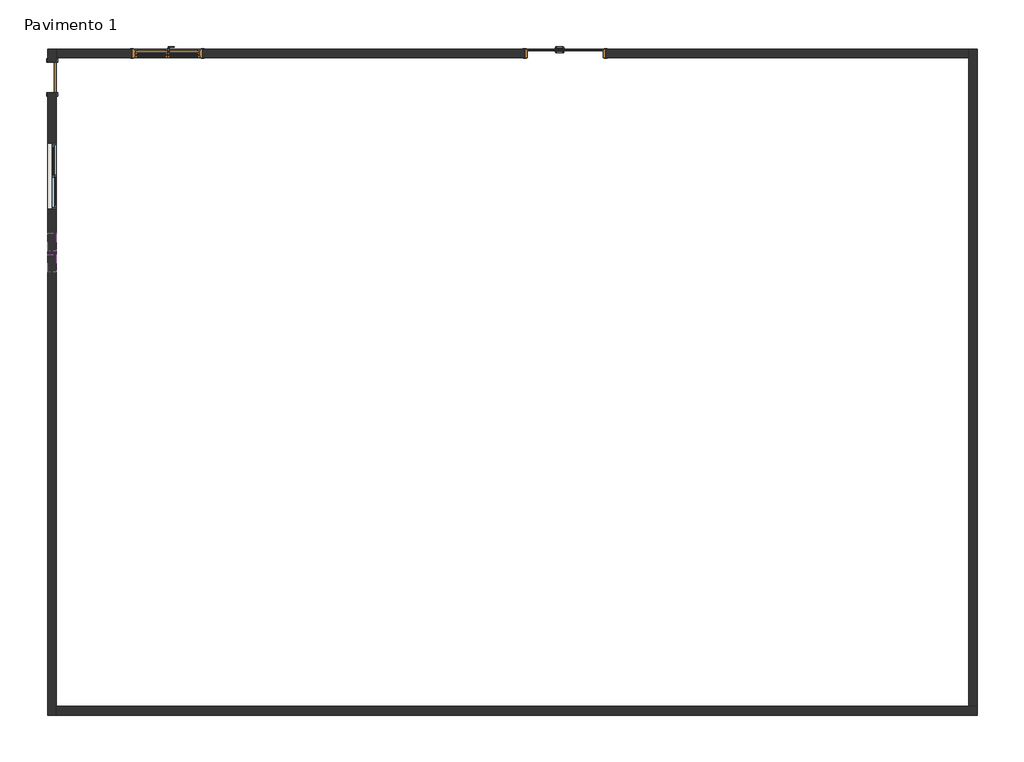
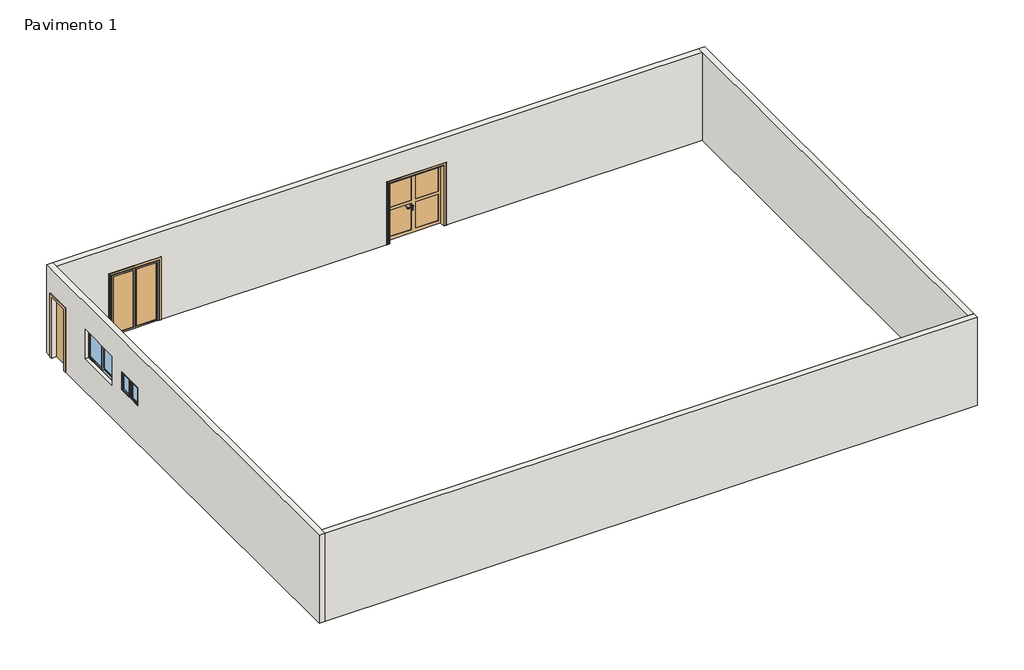
# One storey: 4 walls, 3 doors, 3 windows.
"""IFC4 building model written with IfcOpenShell, lengths in millimetres."""

import ifcopenshell
import ifcopenshell.guid

model = None  # the IFC model being written
_history = None  # IfcOwnerHistory: only IFC2X3 demands one
_inside = {}  # id of a spatial element -> (the spatial element, [elements in it])
_under = {}  # id of a project, library or spatial element -> (it, [spatial elements below it])
_declared = {}  # id of a project -> (the project, [libraries it declares])
_typed = {}  # id of a type object -> (the type object, [elements of that type])
_made_of = {}  # id of a material, layer set ... -> (it, [elements and type objects made of it])


def new_model(schema):
    """Start an empty IFC model of exactly this schema.

    Asked for "IFC4X3", IfcOpenShell would pick the latest addendum, in which some entities
    have other attributes; the version numbers below select the first issue.
    IFC2X3 requires an IfcOwnerHistory on every rooted entity: one is made here for all.
    """
    global model, _history
    if schema == "IFC4X3":
        model = ifcopenshell.file(schema_version=(4, 3, 0, 0))
    else:
        model = ifcopenshell.file(schema=schema)
    _inside.clear()
    _under.clear()
    _declared.clear()
    _typed.clear()
    _made_of.clear()
    _history = None
    if model.schema == "IFC2X3":
        org = make("IfcOrganization", Name="unknown")
        user = make(
            "IfcPersonAndOrganization",
            ThePerson=make("IfcPerson", FamilyName="unknown"),
            TheOrganization=org,
        )
        app = make(
            "IfcApplication",
            ApplicationDeveloper=org,
            Version="unknown",
            ApplicationFullName="unknown",
            ApplicationIdentifier="unknown",
        )
        _history = make(
            "IfcOwnerHistory",
            OwningUser=user,
            OwningApplication=app,
            ChangeAction="ADDED",
            CreationDate=0,
        )
    return model


def make(cls, **values):
    """One entity of the class cls with the attributes given. An attribute that is None is left unset."""
    return model.create_entity(
        cls, **{name: value for name, value in values.items() if value is not None}
    )


def rooted(cls, **values):
    """An entity with a GlobalId (a new one), such as an element, a storey or a relation."""
    return make(cls, GlobalId=ifcopenshell.guid.new(), OwnerHistory=_history, **values)


def si_unit(unit_type, name, prefix=None):
    """IfcSIUnit, for example si_unit("LENGTHUNIT", "METRE", prefix="MILLI")."""
    return make("IfcSIUnit", UnitType=unit_type, Prefix=prefix, Name=name)


def assignment(units):
    """IfcUnitAssignment: the units of a project."""
    return None if units is None else make("IfcUnitAssignment", Units=units)


def point(xyz):
    """IfcCartesianPoint."""
    return None if xyz is None else make("IfcCartesianPoint", Coordinates=xyz)


def direction(xyz):
    """IfcDirection."""
    return None if xyz is None else make("IfcDirection", DirectionRatios=xyz)


def frame(location, z_axis=None, x_axis=None):
    """IfcAxis2Placement3D, a coordinate frame: its origin and axes. An axis left out is left unset."""
    return make(
        "IfcAxis2Placement3D",
        Location=point(location),
        Axis=direction(z_axis),
        RefDirection=direction(x_axis),
    )


def frame_2d(location, x_axis=None):
    """IfcAxis2Placement2D, a coordinate frame in the plane: its origin and x axis."""
    return make(
        "IfcAxis2Placement2D", Location=point(location), RefDirection=direction(x_axis)
    )


def origin():
    """The frame at (0, 0, 0) with its axes left unset."""
    return frame((0.0, 0.0, 0.0))


def origin_with_axes():
    """The frame at (0, 0, 0) with the z axis (0, 0, 1) and the x axis (1, 0, 0) written out."""
    return frame((0.0, 0.0, 0.0), z_axis=(0.0, 0.0, 1.0), x_axis=(1.0, 0.0, 0.0))


def place(relative_to, where):
    """IfcLocalPlacement: puts the frame where relative to a parent placement (None: the world)."""
    return make(
        "IfcLocalPlacement", PlacementRelTo=relative_to, RelativePlacement=where
    )


def context(
    kind, dimensions, precision=None, world=None, true_north=None, identifier=None
):
    """IfcGeometricRepresentationContext, for example the 3D "Model" context."""
    return make(
        "IfcGeometricRepresentationContext",
        ContextIdentifier=identifier,
        ContextType=kind,
        CoordinateSpaceDimension=dimensions,
        Precision=precision,
        WorldCoordinateSystem=world,
        TrueNorth=true_north,
    )


def project(units=None, contexts=None):
    """IfcProject with its units and contexts."""
    return rooted(
        "IfcProject",
        Name="project",
        RepresentationContexts=contexts,
        UnitsInContext=assignment(units),
    )


def spatial(cls, under=None, at=None, **own):
    """A site, building, storey or space (cls), placed at a placement, below another one or the project."""
    s = rooted(cls, ObjectPlacement=at, **own)
    if under is not None:
        _under.setdefault(under.id(), (under, []))[1].append(s)
    return s


def polyline(points):
    """IfcPolyline through the points."""
    return make("IfcPolyline", Points=[point(p) for p in points])


def circle_curve(where, radius):
    """IfcCircle in the frame where."""
    return make("IfcCircle", Position=where, Radius=radius)


def ellipse_curve(where, semi_axis1, semi_axis2):
    """IfcEllipse in the frame where."""
    return make(
        "IfcEllipse", Position=where, SemiAxis1=semi_axis1, SemiAxis2=semi_axis2
    )


def trimmed(basis, trim1, trim2, sense, master):
    """IfcTrimmedCurve: the piece of a basis curve between two trims."""
    return make(
        "IfcTrimmedCurve",
        BasisCurve=basis,
        Trim1=trim1,
        Trim2=trim2,
        SenseAgreement=sense,
        MasterRepresentation=master,
    )


def segment(curve, same_sense, transition):
    """IfcCompositeCurveSegment."""
    return make(
        "IfcCompositeCurveSegment",
        Transition=transition,
        SameSense=same_sense,
        ParentCurve=curve,
    )


def composite_curve(segments, self_intersect=None):
    """IfcCompositeCurve: segments joined end to end."""
    return make("IfcCompositeCurve", Segments=segments, SelfIntersect=self_intersect)


def outline(outer, holes=None, kind="AREA"):
    """IfcArbitraryClosedProfileDef: a profile drawn as a closed curve; with holes, ...WithVoids."""
    if holes is None:
        return make("IfcArbitraryClosedProfileDef", ProfileType=kind, OuterCurve=outer)
    return make(
        "IfcArbitraryProfileDefWithVoids",
        ProfileType=kind,
        OuterCurve=outer,
        InnerCurves=holes,
    )


def extrude(swept, where, along, depth):
    """IfcExtrudedAreaSolid: the profile swept, set in the frame where, extruded along a direction by depth."""
    return make(
        "IfcExtrudedAreaSolid",
        SweptArea=swept,
        Position=where,
        ExtrudedDirection=direction(along),
        Depth=depth,
    )


def faces_of(points, faces, orient=None, outer=None):
    """IfcFace entities. A face is a list of loops; a loop is a list of indices into points, from 0.

    orient and outer hold one flag for each loop. By default every Orientation is true, the
    first loop of a face is its IfcFaceOuterBound and the others are IfcFaceBound.
    """
    made = []
    for i, loops in enumerate(faces):
        bounds = []
        for j, loop in enumerate(loops):
            is_outer = j == 0 if outer is None else outer[i][j]
            bounds.append(
                make(
                    "IfcFaceOuterBound" if is_outer else "IfcFaceBound",
                    Bound=make("IfcPolyLoop", Polygon=[points[k] for k in loop]),
                    Orientation=True if orient is None else orient[i][j],
                )
            )
        made.append(make("IfcFace", Bounds=bounds))
    return made


def faceted_brep(points, faces, orient=None, outer=None, voids=None):
    """IfcFacetedBrep: a solid bounded by flat faces; with voids (closed shells), ...WithVoids."""
    shared = [point(p) for p in points]
    hull = make("IfcClosedShell", CfsFaces=faces_of(shared, faces, orient, outer))
    if voids is None:
        return make("IfcFacetedBrep", Outer=hull)
    return make(
        "IfcFacetedBrepWithVoids",
        Outer=hull,
        Voids=[
            make(cls, CfsFaces=faces_of(shared, fs, o, b)) for cls, fs, o, b in voids
        ],
    )


def shape(context_of_items, identifier, shape_type, items):
    """IfcShapeRepresentation: the items that make up one representation, for example the "Body"."""
    return make(
        "IfcShapeRepresentation",
        ContextOfItems=context_of_items,
        RepresentationIdentifier=identifier,
        RepresentationType=shape_type,
        Items=items,
    )


def source(mapping_origin, context_of_items, identifier, shape_type, items):
    """IfcRepresentationMap: a shape defined once, which mapped items show again and again."""
    return make(
        "IfcRepresentationMap",
        MappingOrigin=mapping_origin,
        MappedRepresentation=shape(context_of_items, identifier, shape_type, items),
    )


def transform(
    local_origin,
    x_axis=None,
    y_axis=None,
    z_axis=None,
    scale=None,
    scale2=None,
    scale3=None,
    uniform=True,
):
    """IfcCartesianTransformationOperator3D, or its non-uniform kind. x_axis, y_axis, z_axis: its Axis1, 2, 3."""
    if uniform:
        return make(
            "IfcCartesianTransformationOperator3D",
            Axis1=direction(x_axis),
            Axis2=direction(y_axis),
            LocalOrigin=point(local_origin),
            Scale=scale,
            Axis3=direction(z_axis),
        )
    return make(
        "IfcCartesianTransformationOperator3DnonUniform",
        Axis1=direction(x_axis),
        Axis2=direction(y_axis),
        LocalOrigin=point(local_origin),
        Scale=scale,
        Axis3=direction(z_axis),
        Scale2=scale2,
        Scale3=scale3,
    )


def mapped(mapping_source, mapping_target):
    """IfcMappedItem: shows the shape of a source again, moved by a transform."""
    return make(
        "IfcMappedItem", MappingSource=mapping_source, MappingTarget=mapping_target
    )


def made_of(thing, what):
    """Note that an element or type object is made of a material, layer set ...; save() writes the relation."""
    if what is not None:
        _made_of.setdefault(what.id(), (what, []))[1].append(thing)
    return thing


def element(
    cls,
    number,
    at=None,
    inside=None,
    cuts=None,
    type_object=None,
    material=None,
    context=None,
    identifier="Body",
    shape_type=None,
    held_by="IfcProductDefinitionShape",
    body=None,
    shapes=None,
    **own,
):
    """One element of the class cls, such as IfcWall. Its Tag is "e" and its number.

    at: its placement. inside: the storey or other place that contains it. cuts: it is an
    opening in that element (IfcRelVoidsElement). A single representation is given by context,
    identifier, shape_type and body (its items); several are given by shapes. held_by: the class
    of the entity that holds the representations. save() writes the other relations.
    """
    e = rooted(cls, Tag="e%d" % number, ObjectPlacement=at, **own)
    if body is not None:
        shapes = [shape(context, identifier, shape_type, body)]
    if shapes is not None:
        e.Representation = make(held_by, Representations=shapes)
    if inside is not None:
        _inside.setdefault(inside.id(), (inside, []))[1].append(e)
    if cuts is not None:
        rooted(
            "IfcRelVoidsElement", RelatingBuildingElement=cuts, RelatedOpeningElement=e
        )
    if type_object is not None:
        _typed.setdefault(type_object.id(), (type_object, []))[1].append(e)
    return made_of(e, material)


def aggregate(whole, parts):
    """IfcRelAggregates: a whole, such as a stair, and the parts it consists of."""
    return rooted("IfcRelAggregates", RelatingObject=whole, RelatedObjects=parts)


def save(model, path):
    """Write the relations noted so far, then the file.

    IfcRelAggregates (storeys below a building ...), IfcRelContainedInSpatialStructure (elements
    in a storey), IfcRelDefinesByType, IfcRelAssociatesMaterial and IfcRelDeclares: one each for
    every whole, place, type object, material and project.
    """
    for whole, parts in _under.values():
        aggregate(whole, parts)
    for where, things in _inside.values():
        rooted(
            "IfcRelContainedInSpatialStructure",
            RelatedElements=things,
            RelatingStructure=where,
        )
    for kind, things in _typed.values():
        rooted("IfcRelDefinesByType", RelatedObjects=things, RelatingType=kind)
    for what, things in _made_of.values():
        rooted("IfcRelAssociatesMaterial", RelatedObjects=things, RelatingMaterial=what)
    for by, libraries in _declared.values():
        rooted("IfcRelDeclares", RelatingContext=by, RelatedDefinitions=libraries)
    model.write(path)


def plane_surface(at):
    """IfcPlane: the flat surface through the origin of the frame at, square to its z axis."""
    return make("IfcPlane", Position=at)


def cylinder_surface(at, radius):
    """IfcCylindricalSurface: all points at the distance radius from the z axis of the frame at."""
    return make("IfcCylindricalSurface", Position=at, Radius=radius)


def revolved_surface(curve, axis_point, axis_direction):
    """IfcSurfaceOfRevolution: the curve turned about the line through axis_point along axis_direction."""
    return make(
        "IfcSurfaceOfRevolution",
        SweptCurve=make("IfcArbitraryOpenProfileDef", ProfileType="CURVE", Curve=curve),
        AxisPosition=make("IfcAxis1Placement", Location=point(axis_point), Axis=direction(axis_direction)),
    )


def advanced_brep(points, edges, surfaces, faces):
    """IfcAdvancedBrep: a solid bounded by faces that lie on surfaces and meet in shared edges.

    An edge is (start, end): straight between two places in points (the first is 0);
    or (start, end, curve); or (start, end, curve, False) where it runs against its curve.
    A face is (place in surfaces, loops), or (place, loops, False) where it looks against
    its surface's normal. A loop lists edges by number (the first is 1), with a minus sign
    where the edge is run from its end to its start. The first loop is the outer one.
    """
    corners = [point(p) for p in points]
    vertices = [make("IfcVertexPoint", VertexGeometry=c) for c in corners]
    made = []
    for start, end, *more in edges:
        made.append(
            make(
                "IfcEdgeCurve",
                EdgeStart=vertices[start],
                EdgeEnd=vertices[end],
                EdgeGeometry=more[0] if more else make("IfcPolyline", Points=[corners[start], corners[end]]),
                SameSense=more[1] if len(more) > 1 else True,
            )
        )
    hull = []
    for where, loops, *sense in faces:
        bounds = []
        for j, loop in enumerate(loops):
            ring = [make("IfcOrientedEdge", EdgeElement=made[abs(k) - 1], Orientation=k > 0) for k in loop]
            bounds.append(
                make(
                    "IfcFaceOuterBound" if j == 0 else "IfcFaceBound",
                    Bound=make("IfcEdgeLoop", EdgeList=ring),
                    Orientation=True,
                )
            )
        hull.append(make("IfcAdvancedFace", Bounds=bounds, FaceSurface=surfaces[where], SameSense=sense[0] if sense else True))
    return make("IfcAdvancedBrep", Outer=make("IfcClosedShell", CfsFaces=hull))


def porta_210x070_b827da78(model_context):
    return source(origin(), model_context, "Body", "SweptSolid", [
        extrude(outline(polyline([(2176.0, -426.0), (0.0, -426.0), (0.0, -350.0), (2100.0, -350.0), (2100.0, 350.0), (0.0, 350.0), (0.0, 426.0), (2176.0, 426.0), (2176.0, -426.0)])), frame((0.0, -125.0, 0.0), z_axis=(0.0, 1.0, 0.0), x_axis=(0.0, 0.0, 1.0)), (0.0, 0.0, 1.0), 25.0),
        extrude(outline(polyline([(2176.0, 426.0), (2176.0, -426.0), (0.0, -426.0), (0.0, -350.0), (2100.0, -350.0), (2100.0, 350.0), (0.0, 350.0), (0.0, 426.0), (2176.0, 426.0)])), frame((0.0, 100.0, 0.0), z_axis=(0.0, 1.0, 0.0), x_axis=(0.0, 0.0, 1.0)), (0.0, 0.0, 1.0), 25.0),
        extrude(outline(polyline([(350.0, -49.0), (350.0, -100.0), (-350.0, -100.0), (-350.0, -49.0), (350.0, -49.0)])), origin_with_axes(), (0.0, 0.0, 1.0), 2100.0),
    ])


def porta_160x210_6cb1d5fe(model_context):
    return source(origin(), model_context, "Body", "SolidModel", [
        extrude(outline(polyline([(-680.0, -7.0), (-680.0, 7.0), (-50.0, 7.0), (-50.0, -7.0), (-680.0, -7.0)])), frame((0.0, 0.0, 50.0), z_axis=(0.0, 0.0, 1.0), x_axis=(1.0, 0.0, 0.0)), (0.0, 0.0, 1.0), 1930.0),
        extrude(outline(polyline([(2030.0, -730.0), (0.0, -730.0), (0.0, 0.0), (2030.0, 0.0), (2030.0, -730.0)]), holes=[polyline([(50.0, -680.0), (1980.0, -680.0), (1980.0, -50.0), (50.0, -50.0), (50.0, -680.0)])]), frame((0.0, -20.0, 0.0), z_axis=(0.0, 1.0, 0.0), x_axis=(0.0, 0.0, 1.0)), (0.0, 0.0, 1.0), 40.0),
        extrude(outline(polyline([(680.0, -7.0), (50.0, -7.0), (50.0, 7.0), (680.0, 7.0), (680.0, -7.0)])), frame((0.0, 0.0, 50.0), z_axis=(0.0, 0.0, 1.0), x_axis=(1.0, 0.0, 0.0)), (0.0, 0.0, 1.0), 1930.0),
        extrude(outline(polyline([(2030.0, 730.0), (2030.0, 0.0), (0.0, 0.0), (0.0, 730.0), (2030.0, 730.0)]), holes=[polyline([(50.0, 680.0), (50.0, 50.0), (1980.0, 50.0), (1980.0, 680.0), (50.0, 680.0)])]), frame((0.0, -20.0, 0.0), z_axis=(0.0, 1.0, 0.0), x_axis=(0.0, 0.0, 1.0)), (0.0, 0.0, 1.0), 40.0),
        extrude(outline(polyline([(-50.0, 89.0), (-50.0, 65.0), (-687.0, 65.0), (-687.0, 89.0), (-50.0, 89.0)])), frame((0.0, 0.0, 53.0), z_axis=(0.0, 0.0, 1.0), x_axis=(1.0, 0.0, 0.0)), (0.0, 0.0, 1.0), 1934.0),
        extrude(outline(polyline([(2037.0, -737.0), (3.0, -737.0), (3.0, 0.0), (2037.0, 0.0), (2037.0, -737.0)]), holes=[polyline([(53.0, -687.0), (1987.0, -687.0), (1987.0, -50.0), (53.0, -50.0), (53.0, -687.0)])]), frame((0.0, 57.0, 0.0), z_axis=(0.0, 1.0, 0.0), x_axis=(0.0, 0.0, 1.0)), (0.0, 0.0, 1.0), 40.0),
        extrude(outline(composite_curve([segment(trimmed(circle_curve(frame_2d((840.0, 25.0)), 15.0), [point((840.0, 40.0))], [point((840.0, 10.0))], False, "CARTESIAN"), True, "CONTINUOUS"), segment(trimmed(circle_curve(frame_2d((840.0, 25.0)), 15.0), [point((840.0, 10.0))], [point((840.0, 40.0))], False, "CARTESIAN"), True, "CONTINUOUS")], self_intersect=False)), frame((0.0, 107.0, 0.0), z_axis=(0.0, 1.0, 0.0), x_axis=(0.0, 0.0, 1.0)), (0.0, 0.0, 1.0), 10.0),
        extrude(outline(composite_curve([segment(trimmed(circle_curve(frame_2d((840.0, 25.0)), 15.0), [point((840.0, 40.0))], [point((840.0, 10.0))], False, "CARTESIAN"), True, "CONTINUOUS"), segment(trimmed(circle_curve(frame_2d((840.0, 25.0)), 15.0), [point((840.0, 10.0))], [point((840.0, 40.0))], False, "CARTESIAN"), True, "CONTINUOUS")], self_intersect=False)), frame((0.0, 37.0, 0.0), z_axis=(0.0, 1.0, 0.0), x_axis=(0.0, 0.0, 1.0)), (0.0, 0.0, 1.0), 10.0),
        extrude(outline(composite_curve([segment(trimmed(circle_curve(frame_2d((900.0, 25.0)), 8.0), [point((904.6523287, 18.4918637))], [point((900.0, 33.0))], False, "CARTESIAN"), True, "CONTINUOUS"), segment(trimmed(circle_curve(frame_2d((894.8738613, 50.3861901)), 18.1261387), [point((900.0, 33.0))], [point((913.0, 50.3861901))], True, "CARTESIAN"), True, "CONTINUOUS"), segment(polyline([(913.0, 50.3861901), (913.0, 126.6435909)]), True, "CONTINUOUS"), segment(trimmed(circle_curve(frame_2d((972.2709207, 123.0603388)), 59.3791355), [point((913.0, 126.6435909))], [point((922.2135558, 155.0))], False, "CARTESIAN"), True, "CONTINUOUS"), segment(polyline([(922.2135558, 155.0), (925.0, 155.0)]), True, "CONTINUOUS"), segment(trimmed(circle_curve(frame_2d((1003.2850638, 126.5772091)), 83.2850902), [point((925.0, 155.0))], [point((920.0, 126.6435909))], True, "CARTESIAN"), True, "CONTINUOUS"), segment(polyline([(920.0, 126.6435909), (920.0, 50.3674333)]), True, "CONTINUOUS"), segment(trimmed(circle_curve(frame_2d((882.7555521, 48.6675129)), 37.2832219), [point((920.0, 50.3674333))], [point((904.6523287, 18.4918637))], False, "CARTESIAN"), True, "CONTINUOUS")], self_intersect=False)), frame((0.0, 137.0, 0.0), z_axis=(0.0, 1.0, 0.0), x_axis=(0.0, 0.0, 1.0)), (0.0, 0.0, 1.0), 20.0),
        extrude(outline(composite_curve([segment(trimmed(circle_curve(frame_2d((894.8738682, 50.3861878)), 18.1261318), [point((899.9999903, 33.0))], [point((913.0, 50.3861878))], True, "CARTESIAN"), True, "CONTINUOUS"), segment(polyline([(913.0, 50.3861878), (913.0, 126.6435909)]), True, "CONTINUOUS"), segment(trimmed(circle_curve(frame_2d((972.2709207, 123.0603388)), 59.3791355), [point((913.0, 126.6435909))], [point((922.2135558, 155.0))], False, "CARTESIAN"), True, "CONTINUOUS"), segment(polyline([(922.2135558, 155.0), (925.0, 155.0)]), True, "CONTINUOUS"), segment(trimmed(circle_curve(frame_2d((1003.2850638, 126.5772091)), 83.2850902), [point((925.0, 155.0))], [point((920.0, 126.6435909))], True, "CARTESIAN"), True, "CONTINUOUS"), segment(polyline([(920.0, 126.6435909), (920.0, 50.3674333)]), True, "CONTINUOUS"), segment(trimmed(circle_curve(frame_2d((882.7555521, 48.6675129)), 37.2832219), [point((920.0, 50.3674333))], [point((904.6523287, 18.4918637))], False, "CARTESIAN"), True, "CONTINUOUS"), segment(trimmed(circle_curve(frame_2d((900.0, 25.0)), 8.0), [point((904.6523287, 18.4918637))], [point((899.9999903, 33.0))], False, "CARTESIAN"), True, "CONTINUOUS")], self_intersect=False)), frame((0.0, -3.0, 0.0), z_axis=(0.0, 1.0, 0.0), x_axis=(0.0, 0.0, 1.0)), (0.0, 0.0, 1.0), 20.0),
        extrude(outline(composite_curve([segment(trimmed(circle_curve(frame_2d((900.0, 25.0)), 8.0), [point((900.0, 33.0))], [point((900.0, 17.0))], False, "CARTESIAN"), True, "CONTINUOUS"), segment(trimmed(circle_curve(frame_2d((900.0, 25.0)), 8.0), [point((900.0, 17.0))], [point((900.0, 33.0))], False, "CARTESIAN"), True, "CONTINUOUS")], self_intersect=False)), frame((0.0, 107.0, 0.0), z_axis=(0.0, 1.0, 0.0), x_axis=(0.0, 0.0, 1.0)), (0.0, 0.0, 1.0), 30.0),
        extrude(outline(composite_curve([segment(trimmed(circle_curve(frame_2d((900.0, 25.0)), 8.0), [point((900.0, 33.0))], [point((900.0, 17.0))], False, "CARTESIAN"), True, "CONTINUOUS"), segment(trimmed(circle_curve(frame_2d((900.0, 25.0)), 8.0), [point((900.0, 17.0))], [point((900.0, 33.0))], False, "CARTESIAN"), True, "CONTINUOUS")], self_intersect=False)), frame((0.0, 17.0, 0.0), z_axis=(0.0, 1.0, 0.0), x_axis=(0.0, 0.0, 1.0)), (0.0, 0.0, 1.0), 30.0),
        extrude(outline(composite_curve([segment(trimmed(circle_curve(frame_2d((830.0, 25.0)), 25.0), [point((830.0, 0.0))], [point((830.0, 50.0))], False, "CARTESIAN"), True, "CONTINUOUS"), segment(polyline([(830.0, 50.0), (900.0, 50.0)]), True, "CONTINUOUS"), segment(trimmed(circle_curve(frame_2d((900.0, 25.0)), 25.0), [point((900.0, 50.0))], [point((900.0, 0.0))], False, "CARTESIAN"), True, "CONTINUOUS"), segment(polyline([(900.0, 0.0), (830.0, 0.0)]), True, "CONTINUOUS")], self_intersect=False)), frame((0.0, 97.0, 0.0), z_axis=(0.0, 1.0, 0.0), x_axis=(0.0, 0.0, 1.0)), (0.0, 0.0, 1.0), 10.0),
        extrude(outline(composite_curve([segment(trimmed(circle_curve(frame_2d((830.0, 25.0)), 25.0), [point((830.0, 0.0))], [point((830.0, 50.0))], False, "CARTESIAN"), True, "CONTINUOUS"), segment(polyline([(830.0, 50.0), (900.0, 50.0)]), True, "CONTINUOUS"), segment(trimmed(circle_curve(frame_2d((900.0, 25.0)), 25.0), [point((900.0, 50.0))], [point((900.0, 0.0))], False, "CARTESIAN"), True, "CONTINUOUS"), segment(polyline([(900.0, 0.0), (830.0, 0.0)]), True, "CONTINUOUS")], self_intersect=False)), frame((0.0, 47.0, 0.0), z_axis=(0.0, 1.0, 0.0), x_axis=(0.0, 0.0, 1.0)), (0.0, 0.0, 1.0), 10.0),
        extrude(outline(polyline([(50.0, 89.0), (687.0, 89.0), (687.0, 65.0), (50.0, 65.0), (50.0, 89.0)])), frame((0.0, 0.0, 53.0), z_axis=(0.0, 0.0, 1.0), x_axis=(1.0, 0.0, 0.0)), (0.0, 0.0, 1.0), 1934.0),
        extrude(outline(polyline([(2037.0, 737.0), (2037.0, 0.0), (3.0, 0.0), (3.0, 737.0), (2037.0, 737.0)]), holes=[polyline([(53.0, 687.0), (53.0, 50.0), (1987.0, 50.0), (1987.0, 687.0), (53.0, 687.0)])]), frame((0.0, 57.0, 0.0), z_axis=(0.0, 1.0, 0.0), x_axis=(0.0, 0.0, 1.0)), (0.0, 0.0, 1.0), 40.0),
        extrude(outline(polyline([(-50.0, -84.0), (-687.0, -84.0), (-687.0, -70.0), (-50.0, -70.0), (-50.0, -84.0)])), frame((0.0, 0.0, 53.0), z_axis=(0.0, 0.0, 1.0), x_axis=(1.0, 0.0, 0.0)), (0.0, 0.0, 1.0), 1934.0),
        extrude(outline(polyline([(3.0, -737.0), (3.0, 0.0), (2037.0, 0.0), (2037.0, -737.0), (3.0, -737.0)]), holes=[polyline([(1987.0, -687.0), (1987.0, -50.0), (53.0, -50.0), (53.0, -687.0), (1987.0, -687.0)])]), frame((0.0, -97.0, 0.0), z_axis=(0.0, 1.0, 0.0), x_axis=(0.0, 0.0, 1.0)), (0.0, 0.0, 1.0), 40.0),
        extrude(outline(polyline([(50.0, -84.0), (50.0, -70.0), (687.0, -70.0), (687.0, -84.0), (50.0, -84.0)])), frame((0.0, 0.0, 53.0), z_axis=(0.0, 0.0, 1.0), x_axis=(1.0, 0.0, 0.0)), (0.0, 0.0, 1.0), 1934.0),
        extrude(outline(polyline([(3.0, 737.0), (2037.0, 737.0), (2037.0, 0.0), (3.0, 0.0), (3.0, 737.0)]), holes=[polyline([(1987.0, 687.0), (53.0, 687.0), (53.0, 50.0), (1987.0, 50.0), (1987.0, 687.0)])]), frame((0.0, -97.0, 0.0), z_axis=(0.0, 1.0, 0.0), x_axis=(0.0, 0.0, 1.0)), (0.0, 0.0, 1.0), 40.0),
        faceted_brep([(-740.0, -100.0, 0.0), (-800.0, -100.0, 0.0), (-800.0, 100.0, 0.0), (-740.0, 100.0, 0.0), (-740.0, 54.0, 0.0), (-730.0, 54.0, 0.0), (-730.0, -54.0, 0.0), (-740.0, -54.0, 0.0), (-740.0, -100.0, 2040.0), (740.0, -100.0, 2040.0), (740.0, -100.0, 0.0), (800.0, -100.0, 0.0), (800.0, -100.0, 2100.0), (-800.0, -100.0, 2100.0), (-800.0, 100.0, 2100.0), (800.0, 100.0, 2100.0), (800.0, 100.0, 0.0), (740.0, 100.0, 0.0), (740.0, 100.0, 2040.0), (-740.0, 100.0, 2040.0), (-740.0, 54.0, 2040.0), (740.0, 54.0, 2040.0), (740.0, 54.0, 0.0), (730.0, 54.0, 0.0), (730.0, 54.0, 2030.0), (-730.0, 54.0, 2030.0), (-730.0, -54.0, 2030.0), (730.0, -54.0, 2030.0), (730.0, -54.0, 0.0), (740.0, -54.0, 0.0), (740.0, -54.0, 2040.0), (-740.0, -54.0, 2040.0)], [[[0, 1, 2, 3, 4, 5, 6, 7]], [[1, 0, 8, 9, 10, 11, 12, 13]], [[2, 1, 13, 14]], [[3, 2, 14, 15, 16, 17, 18, 19]], [[4, 3, 19, 20]], [[5, 4, 20, 21, 22, 23, 24, 25]], [[6, 5, 25, 26]], [[7, 6, 26, 27, 28, 29, 30, 31]], [[0, 7, 31, 8]], [[10, 29, 28, 23, 22, 17, 16, 11]], [[9, 30, 29, 10]], [[27, 24, 23, 28]], [[21, 18, 17, 22]], [[15, 12, 11, 16]], [[14, 13, 12, 15]], [[20, 19, 18, 21]], [[26, 25, 24, 27]], [[8, 31, 30, 9]]]),
        faceted_brep([(843.0, -104.0, 0.0), (837.0, -110.0, 0.0), (773.0, -110.0, 0.0), (773.0, -100.0, 0.0), (843.0, -100.0, 0.0), (843.0, -104.0, 2143.0), (837.0, -110.0, 2137.0), (-837.0, -110.0, 2137.0), (-837.0, -110.0, 0.0), (-773.0, -110.0, 0.0), (-773.0, -110.0, 2073.0), (773.0, -110.0, 2073.0), (773.0, -100.0, 2073.0), (-773.0, -100.0, 2073.0), (-773.0, -100.0, 0.0), (-843.0, -100.0, 0.0), (-843.0, -100.0, 2143.0), (843.0, -100.0, 2143.0), (-843.0, -104.0, 0.0), (-843.0, -104.0, 2143.0)], [[[0, 1, 2, 3, 4]], [[1, 0, 5, 6]], [[2, 1, 6, 7, 8, 9, 10, 11]], [[3, 2, 11, 12]], [[4, 3, 12, 13, 14, 15, 16, 17]], [[0, 4, 17, 5]], [[18, 15, 14, 9, 8]], [[19, 16, 15, 18]], [[13, 10, 9, 14]], [[7, 19, 18, 8]], [[6, 5, 19, 7]], [[12, 11, 10, 13]], [[5, 17, 16, 19]]]),
        faceted_brep([(843.0, 104.0, 0.0), (843.0, 100.0, 0.0), (773.0, 100.0, 0.0), (773.0, 110.0, 0.0), (837.0, 110.0, 0.0), (843.0, 104.0, 2143.0), (843.0, 100.0, 2143.0), (-843.0, 100.0, 2143.0), (-843.0, 100.0, 0.0), (-773.0, 100.0, 0.0), (-773.0, 100.0, 2073.0), (773.0, 100.0, 2073.0), (773.0, 110.0, 2073.0), (-773.0, 110.0, 2073.0), (-773.0, 110.0, 0.0), (-837.0, 110.0, 0.0), (-837.0, 110.0, 2137.0), (837.0, 110.0, 2137.0), (-843.0, 104.0, 0.0), (-843.0, 104.0, 2143.0)], [[[0, 1, 2, 3, 4]], [[1, 0, 5, 6]], [[2, 1, 6, 7, 8, 9, 10, 11]], [[3, 2, 11, 12]], [[4, 3, 12, 13, 14, 15, 16, 17]], [[0, 4, 17, 5]], [[18, 15, 14, 9, 8]], [[19, 16, 15, 18]], [[13, 10, 9, 14]], [[7, 19, 18, 8]], [[6, 5, 19, 7]], [[12, 11, 10, 13]], [[5, 17, 16, 19]]]),
    ])


def porta_de_entrada_dupla_com_revestimento_1840_x_2100mm_8bed4eb5(model_context):
    return source(origin(), model_context, "Body", "SolidModel", [
        advanced_brep(
        [(52.0, -57.0, 900.0), (28.0, -57.0, 900.0), (52.0, -40.0, 900.0), (28.0, -40.0, 900.0), (55.0, -13.0, 900.0), (55.0, -37.0, 900.0), (195.0, -37.0, 900.0), (195.0, -13.0, 900.0), (222.0, -40.0, 900.0), (198.0, -40.0, 900.0), (198.0, -55.0, 900.0), (222.0, -55.0, 900.0)],
        [
            (0, 1, circle_curve(frame((40.0, -57.0, 900.0), z_axis=(0.0, -1.0, 0.0), x_axis=(-1.0, 0.0, 0.0)), 12.0)),
            (1, 0, circle_curve(frame((40.0, -57.0, 900.0), z_axis=(0.0, -1.0, 0.0), x_axis=(-1.0, 0.0, 0.0)), 12.0)),
            (0, 2),
            (2, 3, circle_curve(frame((40.0, -40.0, 900.0), z_axis=(0.0, -1.0, 0.0), x_axis=(-1.0, 0.0, 0.0)), 12.0)),
            (3, 1),
            (3, 2, circle_curve(frame((40.0, -40.0, 900.0), z_axis=(0.0, -1.0, 0.0), x_axis=(-1.0, 0.0, 0.0)), 12.0)),
            (4, 3, circle_curve(frame((55.0, -40.0, 900.0), z_axis=(0.0, 0.0, 1.0), x_axis=(-1.0, 0.0, 0.0)), 27.0)),
            (2, 5, circle_curve(frame((55.0, -40.0, 900.0), z_axis=(0.0, 0.0, -1.0), x_axis=(-1.0, 0.0, 0.0)), 3.0)),
            (5, 4, circle_curve(frame((55.0, -25.0, 900.0), z_axis=(-1.0, 0.0, 0.0), x_axis=(0.0, 1.0, 0.0)), 12.0)),
            (4, 5, circle_curve(frame((55.0, -25.0, 900.0), z_axis=(-1.0, 0.0, 0.0), x_axis=(0.0, 1.0, 0.0)), 12.0)),
            (5, 6),
            (6, 7, circle_curve(frame((195.0, -25.0, 900.0), z_axis=(-1.0, 0.0, 0.0), x_axis=(0.0, 1.0, 0.0)), 12.0)),
            (7, 4),
            (7, 6, circle_curve(frame((195.0, -25.0, 900.0), z_axis=(-1.0, 0.0, 0.0), x_axis=(0.0, 1.0, 0.0)), 12.0)),
            (8, 7, circle_curve(frame((195.0, -40.0, 900.0), z_axis=(0.0, 0.0, 1.0), x_axis=(0.0, 1.0, 0.0)), 27.0)),
            (6, 9, circle_curve(frame((195.0, -40.0, 900.0), z_axis=(0.0, 0.0, -1.0), x_axis=(0.0, 1.0, 0.0)), 3.0)),
            (9, 8, circle_curve(frame((210.0, -40.0, 900.0), z_axis=(0.0, 1.0, 0.0), x_axis=(1.0, 0.0, 0.0)), 12.0)),
            (8, 9, circle_curve(frame((210.0, -40.0, 900.0), z_axis=(0.0, 1.0, 0.0), x_axis=(1.0, 0.0, 0.0)), 12.0)),
            (10, 11, circle_curve(frame((210.0, -55.0, 900.0), z_axis=(0.0, -1.0, 0.0), x_axis=(1.0, 0.0, 0.0)), 12.0)),
            (11, 10, circle_curve(frame((210.0, -55.0, 900.0), z_axis=(0.0, -1.0, 0.0), x_axis=(1.0, 0.0, 0.0)), 12.0)),
            (9, 10),
            (11, 8),
        ],
        [
            plane_surface(frame((-802.0, -57.0, 1730.0), z_axis=(0.0, -1.0, 0.0), x_axis=(0.0, 0.0, 1.0))),
            cylinder_surface(frame((40.0, -57.0, 900.0), z_axis=(0.0, -1.0, 0.0), x_axis=(-1.0, 0.0, 0.0)), 12.0),
            revolved_surface(trimmed(ellipse_curve(frame((40.0, -40.0, 900.0), z_axis=(0.0, -1.0, 0.0), x_axis=(-1.0, 0.0, 0.0)), 12.0, 12.0), [point((52.0, -40.0, 900.0))], [point((28.0, -40.0, 900.0))], True, "CARTESIAN"), (55.0, -40.0, 1730.0), (0.0, 0.0, -1.0)),
            revolved_surface(trimmed(ellipse_curve(frame((40.0, -40.0, 900.0), z_axis=(0.0, -1.0, 0.0), x_axis=(-1.0, 0.0, 0.0)), 12.0, 12.0), [point((28.0, -40.0, 900.0))], [point((52.0, -40.0, 900.0))], True, "CARTESIAN"), (55.0, -40.0, 1730.0), (0.0, 0.0, -1.0)),
            cylinder_surface(frame((55.0, -25.0, 900.0), z_axis=(-1.0, 0.0, 0.0), x_axis=(0.0, 1.0, 0.0)), 12.0),
            revolved_surface(trimmed(ellipse_curve(frame((195.0, -25.0, 900.0), z_axis=(-1.0, 0.0, 0.0), x_axis=(0.0, 1.0, 0.0)), 12.0, 12.0), [point((195.0, -37.0, 900.0))], [point((195.0, -13.0, 900.0))], True, "CARTESIAN"), (195.0, -40.0, 1730.0), (0.0, 0.0, -1.0)),
            revolved_surface(trimmed(ellipse_curve(frame((195.0, -25.0, 900.0), z_axis=(-1.0, 0.0, 0.0), x_axis=(0.0, 1.0, 0.0)), 12.0, 12.0), [point((195.0, -13.0, 900.0))], [point((195.0, -37.0, 900.0))], True, "CARTESIAN"), (195.0, -40.0, 1730.0), (0.0, 0.0, -1.0)),
            plane_surface(frame((-632.0, -55.0, 1730.0), z_axis=(0.0, -1.0, 0.0), x_axis=(0.0, 0.0, -1.0))),
            cylinder_surface(frame((210.0, -40.0, 900.0), z_axis=(0.0, 1.0, 0.0), x_axis=(1.0, 0.0, 0.0)), 12.0),
        ],
        [
            (0, [[1, 2]]),
            (1, [[-1, 3, 4, 5]]),
            (1, [[-2, -5, 6, -3]]),
            (2, [[7, -4, 8, 9]]),
            (3, [[-8, -6, -7, 10]]),
            (4, [[-9, 11, 12, 13]]),
            (4, [[-10, -13, 14, -11]]),
            (5, [[15, -12, 16, 17]]),
            (6, [[-16, -14, -15, 18]]),
            (7, [[19, 20]]),
            (8, [[-17, 21, -20, 22]]),
            (8, [[-18, -22, -19, -21]]),
        ],
    ),
        extrude(outline(composite_curve([segment(trimmed(circle_curve(frame_2d((780.0, 40.0)), 25.0), [point((780.0, 15.0))], [point((780.0, 65.0))], False, "CARTESIAN"), True, "CONTINUOUS"), segment(trimmed(circle_curve(frame_2d((780.0, 40.0)), 25.0), [point((780.0, 65.0))], [point((780.0, 15.0))], False, "CARTESIAN"), True, "CONTINUOUS")], self_intersect=False)), frame((0.0, -65.0, 0.0), z_axis=(0.0, 1.0, 0.0), x_axis=(0.0, 0.0, 1.0)), (0.0, 0.0, 1.0), 8.0),
        extrude(outline(composite_curve([segment(trimmed(circle_curve(frame_2d((900.0, 40.0)), 25.0), [point((900.0, 15.0))], [point((900.0, 65.0))], False, "CARTESIAN"), True, "CONTINUOUS"), segment(trimmed(circle_curve(frame_2d((900.0, 40.0)), 25.0), [point((900.0, 65.0))], [point((900.0, 15.0))], False, "CARTESIAN"), True, "CONTINUOUS")], self_intersect=False)), frame((0.0, -65.0, 0.0), z_axis=(0.0, 1.0, 0.0), x_axis=(0.0, 0.0, 1.0)), (0.0, 0.0, 1.0), 8.0),
        advanced_brep(
        [(28.0, -108.0, 900.0), (52.0, -108.0, 900.0), (28.0, -125.0, 900.0), (52.0, -125.0, 900.0), (55.0, -128.0, 900.0), (55.0, -152.0, 900.0), (195.0, -152.0, 900.0), (195.0, -128.0, 900.0), (198.0, -125.0, 900.0), (222.0, -125.0, 900.0), (222.0, -110.0, 900.0), (198.0, -110.0, 900.0)],
        [
            (0, 1, circle_curve(frame((40.0, -108.0, 900.0), z_axis=(0.0, 1.0, 0.0), x_axis=(1.0, 0.0, 0.0)), 12.0)),
            (1, 0, circle_curve(frame((40.0, -108.0, 900.0), z_axis=(0.0, 1.0, 0.0), x_axis=(1.0, 0.0, 0.0)), 12.0)),
            (0, 2),
            (2, 3, circle_curve(frame((40.0, -125.0, 900.0), z_axis=(0.0, 1.0, 0.0), x_axis=(1.0, 0.0, 0.0)), 12.0)),
            (3, 1),
            (3, 2, circle_curve(frame((40.0, -125.0, 900.0), z_axis=(0.0, 1.0, 0.0), x_axis=(1.0, 0.0, 0.0)), 12.0)),
            (4, 3, circle_curve(frame((55.0, -125.0, 900.0), z_axis=(0.0, 0.0, -1.0), x_axis=(-1.0, 0.0, 0.0)), 3.0)),
            (2, 5, circle_curve(frame((55.0, -125.0, 900.0), z_axis=(0.0, 0.0, 1.0), x_axis=(-1.0, 0.0, 0.0)), 27.0)),
            (5, 4, circle_curve(frame((55.0, -140.0, 900.0), z_axis=(-1.0, 0.0, 0.0), x_axis=(0.0, 1.0, 0.0)), 12.0)),
            (4, 5, circle_curve(frame((55.0, -140.0, 900.0), z_axis=(-1.0, 0.0, 0.0), x_axis=(0.0, 1.0, 0.0)), 12.0)),
            (5, 6),
            (6, 7, circle_curve(frame((195.0, -140.0, 900.0), z_axis=(-1.0, 0.0, 0.0), x_axis=(0.0, 1.0, 0.0)), 12.0)),
            (7, 4),
            (7, 6, circle_curve(frame((195.0, -140.0, 900.0), z_axis=(-1.0, 0.0, 0.0), x_axis=(0.0, 1.0, 0.0)), 12.0)),
            (8, 7, circle_curve(frame((195.0, -125.0, 900.0), z_axis=(0.0, 0.0, -1.0), x_axis=(0.0, -1.0, 0.0)), 3.0)),
            (6, 9, circle_curve(frame((195.0, -125.0, 900.0), z_axis=(0.0, 0.0, 1.0), x_axis=(0.0, -1.0, 0.0)), 27.0)),
            (9, 8, circle_curve(frame((210.0, -125.0, 900.0), z_axis=(0.0, -1.0, 0.0), x_axis=(-1.0, 0.0, 0.0)), 12.0)),
            (8, 9, circle_curve(frame((210.0, -125.0, 900.0), z_axis=(0.0, -1.0, 0.0), x_axis=(-1.0, 0.0, 0.0)), 12.0)),
            (10, 11, circle_curve(frame((210.0, -110.0, 900.0), z_axis=(0.0, 1.0, 0.0), x_axis=(-1.0, 0.0, 0.0)), 12.0)),
            (11, 10, circle_curve(frame((210.0, -110.0, 900.0), z_axis=(0.0, 1.0, 0.0), x_axis=(-1.0, 0.0, 0.0)), 12.0)),
            (9, 10),
            (11, 8),
        ],
        [
            plane_surface(frame((-802.0, -108.0, 1730.0), z_axis=(0.0, 1.0, 0.0), x_axis=(0.0, 0.0, -1.0))),
            cylinder_surface(frame((40.0, -108.0, 900.0), z_axis=(0.0, 1.0, 0.0), x_axis=(1.0, 0.0, 0.0)), 12.0),
            revolved_surface(trimmed(ellipse_curve(frame((40.0, -125.0, 900.0), z_axis=(0.0, 1.0, 0.0), x_axis=(1.0, 0.0, 0.0)), 12.0, 12.0), [point((28.0, -125.0, 900.0))], [point((52.0, -125.0, 900.0))], True, "CARTESIAN"), (55.0, -125.0, 1730.0), (0.0, 0.0, 1.0)),
            revolved_surface(trimmed(ellipse_curve(frame((40.0, -125.0, 900.0), z_axis=(0.0, 1.0, 0.0), x_axis=(1.0, 0.0, 0.0)), 12.0, 12.0), [point((52.0, -125.0, 900.0))], [point((28.0, -125.0, 900.0))], True, "CARTESIAN"), (55.0, -125.0, 1730.0), (0.0, 0.0, 1.0)),
            cylinder_surface(frame((55.0, -140.0, 900.0), z_axis=(-1.0, 0.0, 0.0), x_axis=(0.0, 1.0, 0.0)), 12.0),
            revolved_surface(trimmed(ellipse_curve(frame((195.0, -140.0, 900.0), z_axis=(-1.0, 0.0, 0.0), x_axis=(0.0, 1.0, 0.0)), 12.0, 12.0), [point((195.0, -152.0, 900.0))], [point((195.0, -128.0, 900.0))], True, "CARTESIAN"), (195.0, -125.0, 1730.0), (0.0, 0.0, 1.0)),
            revolved_surface(trimmed(ellipse_curve(frame((195.0, -140.0, 900.0), z_axis=(-1.0, 0.0, 0.0), x_axis=(0.0, 1.0, 0.0)), 12.0, 12.0), [point((195.0, -128.0, 900.0))], [point((195.0, -152.0, 900.0))], True, "CARTESIAN"), (195.0, -125.0, 1730.0), (0.0, 0.0, 1.0)),
            plane_surface(frame((-632.0, -110.0, 1730.0), z_axis=(0.0, 1.0, 0.0), x_axis=(0.0, 0.0, 1.0))),
            cylinder_surface(frame((210.0, -125.0, 900.0), z_axis=(0.0, -1.0, 0.0), x_axis=(-1.0, 0.0, 0.0)), 12.0),
        ],
        [
            (0, [[1, 2]]),
            (1, [[-1, 3, 4, 5]]),
            (1, [[-2, -5, 6, -3]]),
            (2, [[7, -4, 8, 9]]),
            (3, [[-8, -6, -7, 10]]),
            (4, [[-9, 11, 12, 13]]),
            (4, [[-10, -13, 14, -11]]),
            (5, [[15, -12, 16, 17]]),
            (6, [[-16, -14, -15, 18]]),
            (7, [[19, 20]]),
            (8, [[-17, 21, -20, 22]]),
            (8, [[-18, -22, -19, -21]]),
        ],
    ),
        extrude(outline(composite_curve([segment(trimmed(circle_curve(frame_2d((780.0, 40.0)), 25.0), [point((780.0, 15.0))], [point((780.0, 65.0))], False, "CARTESIAN"), True, "CONTINUOUS"), segment(trimmed(circle_curve(frame_2d((780.0, 40.0)), 25.0), [point((780.0, 65.0))], [point((780.0, 15.0))], False, "CARTESIAN"), True, "CONTINUOUS")], self_intersect=False)), frame((0.0, -108.0, 0.0), z_axis=(0.0, 1.0, 0.0), x_axis=(0.0, 0.0, 1.0)), (0.0, 0.0, 1.0), 8.0),
        extrude(outline(composite_curve([segment(trimmed(circle_curve(frame_2d((900.0, 40.0)), 25.0), [point((900.0, 15.0))], [point((900.0, 65.0))], False, "CARTESIAN"), True, "CONTINUOUS"), segment(trimmed(circle_curve(frame_2d((900.0, 40.0)), 25.0), [point((900.0, 65.0))], [point((900.0, 15.0))], False, "CARTESIAN"), True, "CONTINUOUS")], self_intersect=False)), frame((0.0, -108.0, 0.0), z_axis=(0.0, 1.0, 0.0), x_axis=(0.0, 0.0, 1.0)), (0.0, 0.0, 1.0), 8.0),
        extrude(outline(polyline([(-835.0, -75.5), (835.0, -75.5), (835.0, -89.5), (-835.0, -89.5), (-835.0, -75.5)])), frame((0.0, 0.0, 70.0), z_axis=(0.0, 0.0, 1.0), x_axis=(1.0, 0.0, 0.0)), (0.0, 0.0, 1.0), 970.0),
        extrude(outline(polyline([(-835.0, -75.5), (835.0, -75.5), (835.0, -89.5), (-835.0, -89.5), (-835.0, -75.5)])), frame((0.0, 0.0, 1060.0), z_axis=(0.0, 0.0, 1.0), x_axis=(1.0, 0.0, 0.0)), (0.0, 0.0, 1.0), 955.0),
        extrude(outline(polyline([(-835.0, -75.5), (835.0, -75.5), (835.0, -89.5), (-835.0, -89.5), (-835.0, -75.5)])), frame((0.0, 0.0, 70.0), z_axis=(0.0, 0.0, 1.0), x_axis=(1.0, 0.0, 0.0)), (0.0, 0.0, 1.0), 970.0),
        extrude(outline(polyline([(-835.0, -75.5), (835.0, -75.5), (835.0, -89.5), (-835.0, -89.5), (-835.0, -75.5)])), frame((0.0, 0.0, 1060.0), z_axis=(0.0, 0.0, 1.0), x_axis=(1.0, 0.0, 0.0)), (0.0, 0.0, 1.0), 955.0),
        faceted_brep([(-920.0, 100.0, 0.0), (-870.0, 100.0, 0.0), (-870.0, -62.0, 0.0), (-880.0, -62.0, 0.0), (-880.0, -100.0, 0.0), (-920.0, -100.0, 0.0), (-920.0, 100.0, 2100.0), (920.0, 100.0, 2100.0), (920.0, 100.0, 0.0), (870.0, 100.0, 0.0), (870.0, 100.0, 2050.0), (-870.0, 100.0, 2050.0), (-870.0, -62.0, 2050.0), (870.0, -62.0, 2050.0), (870.0, -62.0, 0.0), (880.0, -62.0, 0.0), (880.0, -62.0, 2060.0), (-880.0, -62.0, 2060.0), (-880.0, -100.0, 2060.0), (880.0, -100.0, 2060.0), (880.0, -100.0, 0.0), (920.0, -100.0, 0.0), (920.0, -100.0, 2100.0), (-920.0, -100.0, 2100.0)], [[[0, 1, 2, 3, 4, 5]], [[1, 0, 6, 7, 8, 9, 10, 11]], [[2, 1, 11, 12]], [[3, 2, 12, 13, 14, 15, 16, 17]], [[4, 3, 17, 18]], [[5, 4, 18, 19, 20, 21, 22, 23]], [[0, 5, 23, 6]], [[7, 22, 21, 8]], [[8, 21, 20, 15, 14, 9]], [[13, 10, 9, 14]], [[19, 16, 15, 20]], [[12, 11, 10, 13]], [[18, 17, 16, 19]], [[6, 23, 22, 7]]]),
        faceted_brep([(963.0, -102.0, 0.0), (957.0, -108.0, 0.0), (893.0, -108.0, 0.0), (893.0, -100.0, 0.0), (963.0, -100.0, 0.0), (963.0, -102.0, 2143.0), (957.0, -108.0, 2137.0), (-957.0, -108.0, 2137.0), (-957.0, -108.0, 0.0), (-893.0, -108.0, 0.0), (-893.0, -108.0, 2073.0), (893.0, -108.0, 2073.0), (893.0, -100.0, 2073.0), (-893.0, -100.0, 2073.0), (-893.0, -100.0, 0.0), (-963.0, -100.0, 0.0), (-963.0, -100.0, 2143.0), (963.0, -100.0, 2143.0), (-963.0, -102.0, 2143.0), (-963.0, -102.0, 0.0)], [[[0, 1, 2, 3, 4]], [[1, 0, 5, 6]], [[2, 1, 6, 7, 8, 9, 10, 11]], [[3, 2, 11, 12]], [[4, 3, 12, 13, 14, 15, 16, 17]], [[0, 4, 17, 5]], [[7, 18, 19, 8]], [[19, 15, 14, 9, 8]], [[13, 10, 9, 14]], [[18, 16, 15, 19]], [[6, 5, 18, 7]], [[12, 11, 10, 13]], [[5, 17, 16, 18]]]),
        faceted_brep([(-963.0, 102.0, 0.0), (-957.0, 108.0, 0.0), (-893.0, 108.0, 0.0), (-893.0, 100.0, 0.0), (-963.0, 100.0, 0.0), (-963.0, 102.0, 2143.0), (-957.0, 108.0, 2137.0), (957.0, 108.0, 2137.0), (957.0, 108.0, 0.0), (893.0, 108.0, 0.0), (893.0, 108.0, 2073.0), (-893.0, 108.0, 2073.0), (-893.0, 100.0, 2073.0), (893.0, 100.0, 2073.0), (893.0, 100.0, 0.0), (963.0, 100.0, 0.0), (963.0, 100.0, 2143.0), (-963.0, 100.0, 2143.0), (963.0, 102.0, 2143.0), (963.0, 102.0, 0.0)], [[[0, 1, 2, 3, 4]], [[1, 0, 5, 6]], [[2, 1, 6, 7, 8, 9, 10, 11]], [[3, 2, 11, 12]], [[4, 3, 12, 13, 14, 15, 16, 17]], [[0, 4, 17, 5]], [[7, 18, 19, 8]], [[19, 15, 14, 9, 8]], [[13, 10, 9, 14]], [[18, 16, 15, 19]], [[6, 5, 18, 7]], [[12, 11, 10, 13]], [[5, 17, 16, 18]]]),
        extrude(outline(polyline([(2060.0, -880.0), (0.0, -880.0), (0.0, 880.0), (2060.0, 880.0), (2060.0, -880.0)]), holes=[polyline([(1975.0, 75.0), (1975.0, 795.0), (1100.0, 795.0), (1100.0, 75.0), (1975.0, 75.0)]), polyline([(1100.0, -795.0), (1975.0, -795.0), (1975.0, -75.0), (1100.0, -75.0), (1100.0, -795.0)]), polyline([(1000.0, 795.0), (110.0, 795.0), (110.0, 75.0), (1000.0, 75.0), (1000.0, 795.0)]), polyline([(110.0, -75.0), (110.0, -795.0), (1000.0, -795.0), (1000.0, -75.0), (110.0, -75.0)])]), frame((0.0, -100.0, 0.0), z_axis=(0.0, 1.0, 0.0), x_axis=(0.0, 0.0, 1.0)), (0.0, 0.0, 1.0), 35.0),
    ])


def window_fbe88107(model_context):
    return source(origin(), model_context, "Body", "SweptSolid", [
        extrude(outline(polyline([(-665.0, -73.0), (-25.0, -73.0), (-25.0, -87.0), (-665.0, -87.0), (-665.0, -73.0)])), frame((0.0, 0.0, 1185.0), z_axis=(0.0, 0.0, 1.0), x_axis=(1.0, 0.0, 0.0)), (0.0, 0.0, 1.0), 830.0),
        extrude(outline(polyline([(25.0, -23.0), (665.0, -23.0), (665.0, -37.0), (25.0, -37.0), (25.0, -23.0)])), frame((0.0, 0.0, 1185.0), z_axis=(0.0, 0.0, 1.0), x_axis=(1.0, 0.0, 0.0)), (0.0, 0.0, 1.0), 830.0),
        extrude(outline(polyline([(2100.0, 750.0), (2100.0, -750.0), (1100.0, -750.0), (1100.0, 750.0), (2100.0, 750.0)]), holes=[polyline([(1135.0, 715.0), (1135.0, -715.0), (2065.0, -715.0), (2065.0, 715.0), (1135.0, 715.0)])]), frame((0.0, -100.0, 0.0), z_axis=(0.0, 1.0, 0.0), x_axis=(0.0, 0.0, 1.0)), (0.0, 0.0, 1.0), 90.0),
        extrude(outline(polyline([(2065.0, 25.0), (2065.0, -715.0), (1135.0, -715.0), (1135.0, 25.0), (2065.0, 25.0)]), holes=[polyline([(1185.0, -25.0), (1185.0, -665.0), (2015.0, -665.0), (2015.0, -25.0), (1185.0, -25.0)])]), frame((0.0, -100.0, 0.0), z_axis=(0.0, 1.0, 0.0), x_axis=(0.0, 0.0, 1.0)), (0.0, 0.0, 1.0), 40.0),
        extrude(outline(polyline([(1135.0, -25.0), (1135.0, 715.0), (2065.0, 715.0), (2065.0, -25.0), (1135.0, -25.0)]), holes=[polyline([(2015.0, 25.0), (2015.0, 665.0), (1185.0, 665.0), (1185.0, 25.0), (2015.0, 25.0)])]), frame((0.0, -50.0, 0.0), z_axis=(0.0, 1.0, 0.0), x_axis=(0.0, 0.0, 1.0)), (0.0, 0.0, 1.0), 40.0),
    ])


def m_fixo_0406_x_0610mm_8205b201(model_context):
    return source(origin(), model_context, "Body", "SweptSolid", [
        extrude(outline(polyline([(-140.0, 78.0), (140.0, 78.0), (140.0, 66.0), (-140.0, 66.0), (-140.0, 78.0)])), frame((0.0, 0.0, 978.0), z_axis=(0.0, 0.0, 1.0), x_axis=(1.0, 0.0, 0.0)), (0.0, 0.0, 1.0), 484.0),
        extrude(outline(polyline([(1506.0, -184.0), (934.0, -184.0), (934.0, 184.0), (1506.0, 184.0), (1506.0, -184.0)]), holes=[polyline([(1462.0, -140.0), (1462.0, 140.0), (978.0, 140.0), (978.0, -140.0), (1462.0, -140.0)])]), frame((0.0, 50.0, 0.0), z_axis=(0.0, 1.0, 0.0), x_axis=(0.0, 0.0, 1.0)), (0.0, 0.0, 1.0), 44.0),
        extrude(outline(polyline([(1525.0, -203.0), (915.0, -203.0), (915.0, 203.0), (1525.0, 203.0), (1525.0, -203.0)]), holes=[polyline([(1506.0, -184.0), (1506.0, 184.0), (934.0, 184.0), (934.0, -184.0), (1506.0, -184.0)])]), frame((0.0, 50.0, 0.0), z_axis=(0.0, 1.0, 0.0), x_axis=(0.0, 0.0, 1.0)), (0.0, 0.0, 1.0), 63.0),
        extrude(outline(polyline([(1525.0, -203.0), (915.0, -203.0), (915.0, 203.0), (1525.0, 203.0), (1525.0, -203.0)]), holes=[polyline([(1493.0, -171.0), (1493.0, 171.0), (947.0, 171.0), (947.0, -171.0), (1493.0, -171.0)])]), frame((0.0, -87.0, 0.0), z_axis=(0.0, 1.0, 0.0), x_axis=(0.0, 0.0, 1.0)), (0.0, 0.0, 1.0), 137.0),
    ])


model = new_model("IFC4")

# Units and contexts
model_context = context("Model", 3, world=origin())
ifc_project = project(units=[si_unit("LENGTHUNIT", "METRE", prefix="MILLI")], contexts=[model_context])

# Site, building, storey
site = spatial("IfcSite", under=ifc_project)
building = spatial("IfcBuilding", under=site)
storey = spatial("IfcBuildingStorey", under=building, Name="Pavimento 1", Elevation=0.0)

# Doors
placement = place(None, origin())
porta_210x070_shape = porta_210x070_b827da78(model_context)
element("IfcDoor", 1, ObjectType="M_Folha única : .Porta - 210x070", at=placement, inside=storey, context=model_context, shape_type="MappedRepresentation", body=[
    mapped(porta_210x070_shape, transform((-10826.104315, 4371.8769454, 0.0), x_axis=(0.0, 1.0, 0.0), y_axis=(-1.0, 0.0, 0.0), z_axis=(0.0, 0.0, 1.0))),
])
porta_160x210_shape = porta_160x210_6cb1d5fe(model_context)
element("IfcDoor", 2, ObjectType="Abertura da porta e vidraça com revestimento : .Porta 160x210", at=placement, inside=storey, context=model_context, shape_type="MappedRepresentation", body=[
    mapped(porta_160x210_shape, transform((-8196.104315, 4921.8769454, 0.0), x_axis=(1.0, 0.0, 0.0), y_axis=(0.0, 1.0, 0.0), z_axis=(0.0, 0.0, 1.0))),
])
porta_de_entrada_dupla_com_revestimento_1840_x_2100mm_shape = porta_de_entrada_dupla_com_revestimento_1840_x_2100mm_8bed4eb5(model_context)
element("IfcDoor", 3, ObjectType="Porta de entrada dupla com revestimento : 1840 x 2100mm", at=placement, inside=storey, context=model_context, shape_type="MappedRepresentation", body=[
    mapped(porta_de_entrada_dupla_com_revestimento_1840_x_2100mm_shape, transform((873.895685, 4921.8769454, 0.0), x_axis=(-1.0, 0.0, 0.0), y_axis=(0.0, -1.0, 0.0), z_axis=(0.0, 0.0, 1.0))),
])

# Walls
element("IfcWall", 4, ObjectType=".Parede 020 cm", at=placement, inside=storey, context=model_context, shape_type="Brep", body=[
    faceted_brep([(-10726.104315, 4721.8769454, 2100.0), (-10726.104315, 4721.8769454, 0.0), (-10726.104315, 4821.8769454, 0.0), (-10726.104315, 5021.8769454, 0.0), (-10726.104315, 5021.8769454, 3000.0), (-10726.104315, 4821.8769454, 3000.0), (-10726.104315, -9978.1230546, 3000.0), (-10726.104315, -10178.1230546, 3000.0), (-10726.104315, -10178.1230546, 0.0), (-10726.104315, -9978.1230546, 0.0), (-10726.104315, 4021.8769454, 0.0), (-10726.104315, 4021.8769454, 2100.0), (-10726.104315, 415.8769454, 1281.6230724), (-10726.104315, 415.8769454, 1891.6230724), (-10726.104315, 821.8769454, 1891.6230724), (-10726.104315, 821.8769454, 1281.6230724), (-10726.104315, -70.1230546, 1284.1484584), (-10726.104315, -70.1230546, 1894.1484584), (-10726.104315, 335.8769454, 1894.1484584), (-10726.104315, 335.8769454, 1284.1484584), (-10726.104315, 1371.8769454, 1100.0), (-10726.104315, 1371.8769454, 2100.0), (-10726.104315, 2871.8769454, 2100.0), (-10726.104315, 2871.8769454, 1100.0), (-10926.104315, 5021.8769454, 0.0), (-10926.104315, 4721.8769454, 0.0), (-10926.104315, 4721.8769454, 2100.0), (-10926.104315, 4021.8769454, 2100.0), (-10926.104315, 4021.8769454, 0.0), (-10926.104315, -10178.1230546, 0.0), (-10926.104315, -10178.1230546, 3000.0), (-10926.104315, 5021.8769454, 3000.0), (-10926.104315, 415.8769454, 1281.6230724), (-10926.104315, 821.8769454, 1281.6230724), (-10926.104315, 821.8769454, 1891.6230724), (-10926.104315, 415.8769454, 1891.6230724), (-10926.104315, -70.1230546, 1284.1484584), (-10926.104315, 335.8769454, 1284.1484584), (-10926.104315, 335.8769454, 1894.1484584), (-10926.104315, -70.1230546, 1894.1484584), (-10926.104315, 1371.8769454, 1100.0), (-10926.104315, 2871.8769454, 1100.0), (-10926.104315, 2871.8769454, 2100.0), (-10926.104315, 1371.8769454, 2100.0)], [[[0, 1, 2, 3, 4, 5, 6, 7, 8, 9, 10, 11], [12, 13, 14, 15], [16, 17, 18, 19], [20, 21, 22, 23]], [[24, 25, 26, 27, 28, 29, 30, 31], [32, 33, 34, 35], [36, 37, 38, 39], [40, 41, 42, 43]], [[10, 9, 8, 29, 28]], [[3, 2, 1, 25, 24]], [[7, 6, 5, 4, 31, 30]], [[8, 7, 30, 29]], [[4, 3, 24, 31]], [[26, 25, 1, 0]], [[27, 26, 0, 11]], [[28, 27, 11, 10]], [[13, 12, 32, 35]], [[14, 13, 35, 34]], [[15, 14, 34, 33]], [[12, 15, 33, 32]], [[17, 16, 36, 39]], [[18, 17, 39, 38]], [[19, 18, 38, 37]], [[16, 19, 37, 36]], [[21, 20, 40, 43]], [[22, 21, 43, 42]], [[23, 22, 42, 41]], [[20, 23, 41, 40]]]),
])
element("IfcWall", 5, ObjectType=".Parede 020 cm", at=placement, inside=storey, context=model_context, shape_type="Brep", body=[
    faceted_brep([(10273.895685, -9978.1230546, 0.0), (10073.895685, -9978.1230546, 0.0), (-10726.104315, -9978.1230546, 0.0), (-10726.104315, -9978.1230546, 3000.0), (10073.895685, -9978.1230546, 3000.0), (10273.895685, -9978.1230546, 3000.0), (10273.895685, -10178.1230546, 0.0), (10273.895685, -10178.1230546, 3000.0), (-10726.104315, -10178.1230546, 3000.0), (-10726.104315, -10178.1230546, 0.0)], [[[0, 1, 2, 3, 4, 5]], [[6, 7, 8, 9]], [[2, 1, 0, 6, 9]], [[5, 4, 3, 8, 7]], [[0, 5, 7, 6]], [[3, 2, 9, 8]]]),
])
element("IfcWall", 6, ObjectType=".Parede 020 cm", at=placement, inside=storey, context=model_context, shape_type="Brep", body=[
    faceted_brep([(10073.895685, 5021.8769454, 0.0), (10073.895685, 4821.8769454, 0.0), (10073.895685, -9978.1230546, 0.0), (10073.895685, -9978.1230546, 3000.0), (10073.895685, 4821.8769454, 3000.0), (10073.895685, 5021.8769454, 3000.0), (10273.895685, 5021.8769454, 0.0), (10273.895685, 5021.8769454, 3000.0), (10273.895685, -9978.1230546, 3000.0), (10273.895685, -9978.1230546, 0.0)], [[[0, 1, 2, 3, 4, 5]], [[6, 7, 8, 9]], [[2, 1, 0, 6, 9]], [[5, 4, 3, 8, 7]], [[3, 2, 9, 8]], [[0, 5, 7, 6]]]),
])
element("IfcWall", 7, ObjectType=".Parede 020 cm", at=placement, inside=storey, context=model_context, shape_type="SweptSolid", body=[
    extrude(outline(polyline([(3000.0, 10073.895685), (3000.0, -10726.104315), (0.0, -10726.104315), (0.0, -8996.104315), (2100.0, -8996.104315), (2100.0, -7396.104315), (0.0, -7396.104315), (0.0, -46.104315), (2100.0, -46.104315), (2100.0, 1793.895685), (0.0, 1793.895685), (0.0, 10073.895685), (3000.0, 10073.895685)])), frame((0.0, 4821.8769454, 0.0), z_axis=(0.0, 1.0, 0.0), x_axis=(0.0, 0.0, 1.0)), (0.0, 0.0, 1.0), 200.0),
])

# Windows
window_shape = window_fbe88107(model_context)
element("IfcWindow", 8, ObjectType="Janela de correr - 2 Painéis : .Janela 2 Folhas - 150x100/110", at=placement, inside=storey, context=model_context, shape_type="MappedRepresentation", body=[
    mapped(window_shape, transform((-10826.104315, 2121.8769454, 0.0), x_axis=(0.0, 1.0, 0.0), y_axis=(-1.0, 0.0, 0.0), z_axis=(0.0, 0.0, 1.0))),
])
m_fixo_0406_x_0610mm_shape = m_fixo_0406_x_0610mm_8205b201(model_context)
element("IfcWindow", 9, ObjectType="M_Fixo : 0406 x 0610mm", at=placement, inside=storey, context=model_context, shape_type="MappedRepresentation", body=[
    mapped(m_fixo_0406_x_0610mm_shape, transform((-10813.104315, 618.8769454, 366.6230724), x_axis=(0.0, 1.0, 0.0), y_axis=(-1.0, 0.0, 0.0), z_axis=(0.0, 0.0, 1.0))),
])
element("IfcWindow", 10, ObjectType="M_Fixo : 0406 x 0610mm", at=placement, inside=storey, context=model_context, shape_type="MappedRepresentation", body=[
    mapped(m_fixo_0406_x_0610mm_shape, transform((-10813.104315, 132.8769454, 369.1484584), x_axis=(0.0, 1.0, 0.0), y_axis=(-1.0, 0.0, 0.0), z_axis=(0.0, 0.0, 1.0))),
])

save(model, "model.ifc")

# Revit data of these elements
# Project information
#   Data de emissão do projeto = "Data de emissão"
#   Status do projeto = "Status do projeto"
#   Nome do cliente = "Proprietário"
#   Endereço do projeto = "Insira aqui o endereço"
#   Nome do projeto = "Nome do projeto"
#   Número do projeto = "0001"
# Type "M_Folha única : .Porta - 210x070"
#   Type Mark = "40"
#   Construction Type Id = "MDOOR"
#   Analytic Construction = "Metal"
#   Thickness = 0.051 m
#   Thermal Resistance (R) = 0.270117 (m²·K)/W
#   Heat Transfer Coefficient (U) = 3.7021 W/(m²·K)
#   Height = 2.10 m
#   Projeção da apara externa = 0.025 m
#   Projeção da apara interna = 0.025 m
#   Largura da apara = 0.076 m
#   Width = 0.70 m
#   Define Thermal Properties by = 1
#   Material da porta = Porta - Painel
#   Material da moldura = Porta - Batente
#   Visual Light Transmittance = 0
#   Solar Heat Gain Coefficient = 0
#   Function = (empty or 0)
#   Wall Closure = (empty or 0)
# Type "Abertura da porta e vidraça com revestimento : .Porta 160x210"
#   Type Mark = "50"
#   Construction Type Id = "MDOOR"
